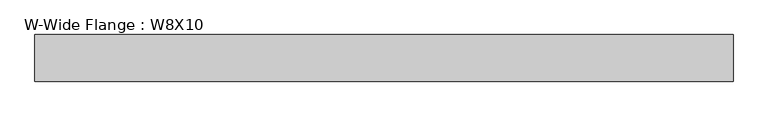
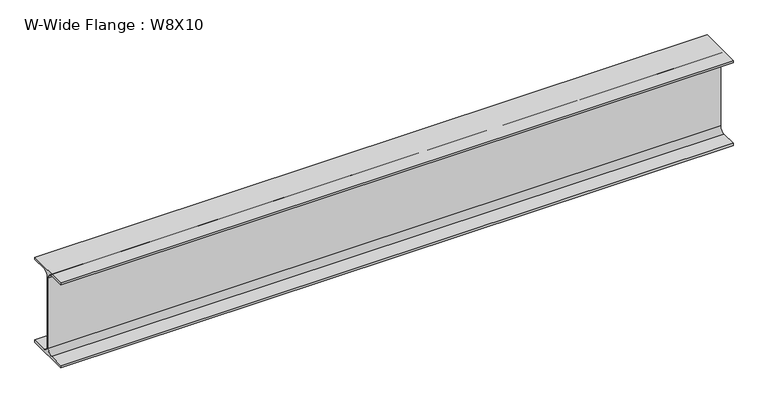
"""IFC4 building model written with IfcOpenShell, lengths in millimetres: beam geometry, W-Wide Flange : W8X10."""

from ifc_helpers import new_model, si_unit, point, frame, frame_2d, origin, place, context, project, spatial, polyline, circle_curve, trimmed, segment, composite_curve, outline, extrude, source, transform, mapped, element, save


def w_wide_flange_w8x10_993dd0ac(model_context):
    return source(origin(), model_context, "Body", "SweptSolid", [
        extrude(outline(composite_curve([segment(polyline([(50.038, -94.996), (50.038, -100.203), (-50.038, -100.203), (-50.038, -94.996), (-14.4145, -94.996)]), True, "CONTINUOUS"), segment(trimmed(circle_curve(frame_2d((-14.4145, -82.7405)), 12.2555), [point((-14.4145, -94.996))], [point((-2.159, -82.7405))], True, "CARTESIAN"), True, "CONTINUOUS"), segment(polyline([(-2.159, -82.7405), (-2.159, 82.7405)]), True, "CONTINUOUS"), segment(trimmed(circle_curve(frame_2d((-14.4145, 82.7405)), 12.2555), [point((-2.159, 82.7405))], [point((-14.4145, 94.996))], True, "CARTESIAN"), True, "CONTINUOUS"), segment(polyline([(-14.4145, 94.996), (-50.038, 94.996), (-50.038, 100.203), (50.038, 100.203), (50.038, 94.996), (14.4145, 94.996)]), True, "CONTINUOUS"), segment(trimmed(circle_curve(frame_2d((14.4145, 82.7405)), 12.2555), [point((14.4145, 94.996))], [point((2.159, 82.7405))], True, "CARTESIAN"), True, "CONTINUOUS"), segment(polyline([(2.159, 82.7405), (2.159, -82.7405)]), True, "CONTINUOUS"), segment(trimmed(circle_curve(frame_2d((14.4145, -82.7405)), 12.2555), [point((2.159, -82.7405))], [point((14.4145, -94.996))], True, "CARTESIAN"), True, "CONTINUOUS"), segment(polyline([(14.4145, -94.996), (50.038, -94.996)]), True, "CONTINUOUS")], self_intersect=False)), frame((-758.825, 0.0, 0.0), z_axis=(1.0, 0.0, 0.0), x_axis=(0.0, 1.0, 0.0)), (0.0, 0.0, 1.0), 1498.8480469),
    ])


if __name__ == "__main__":
    model = new_model("IFC4")
    model_context = context("Model", 3, world=origin())
    ifc_project = project(units=[si_unit("LENGTHUNIT", "METRE", prefix="MILLI")], contexts=[model_context])
    site = spatial("IfcSite", under=ifc_project)
    building = spatial("IfcBuilding", under=site)
    placement = place(None, origin())
    w_wide_flange_w8x10_shape = w_wide_flange_w8x10_993dd0ac(model_context)
    element("IfcBeam", 1, ObjectType="W-Wide Flange : W8X10", at=placement, inside=building, context=model_context, shape_type="MappedRepresentation", body=[
        mapped(w_wide_flange_w8x10_shape, transform((0.0, 0.0, 0.0), x_axis=(1.0, 0.0, 0.0), y_axis=(0.0, 1.0, 0.0), z_axis=(0.0, 0.0, 1.0))),
    ])
    save(model, "model.ifc")

# Revit data of these elements
# Type "W-Wide Flange : W8X10"
#   Assembly Code = "B10"
#   W = 10
#   Length [instance default] = 1524 mm
#   bf = 100.076 mm
#   d = 200.406 mm
#   k = 17.463 mm
#   k2 = 12.255 mm
#   tf = 5.207 mm
#   tw = 4.318 mm
#   A = 0.00190967 m²
#   Structural Material [instance default] = Steel ASTM A992
# Element 1 (IfcBeam, "W-Wide Flange : W8X10")
#   Structural Material = Aluminum, Anodized Red
#   Materials on its faces: "Aluminum, Anodized Red"
# Materials
#   "Steel ASTM A992": class "Metal", colour RGB 128 0 0, transparency 0, Description = "Structural steel 50ksi", Cost = 0
#   "Aluminum, Anodized Red": class "Metal", colour RGB 120 120 120, transparency 0, Description = "Anodized aluminum, red", Cost = 0
